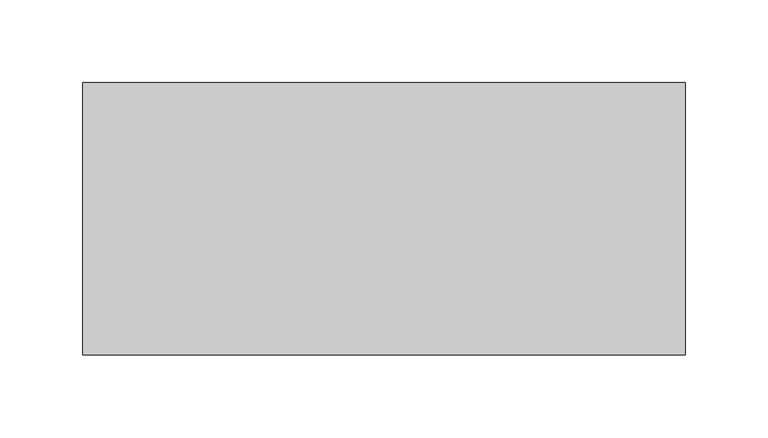
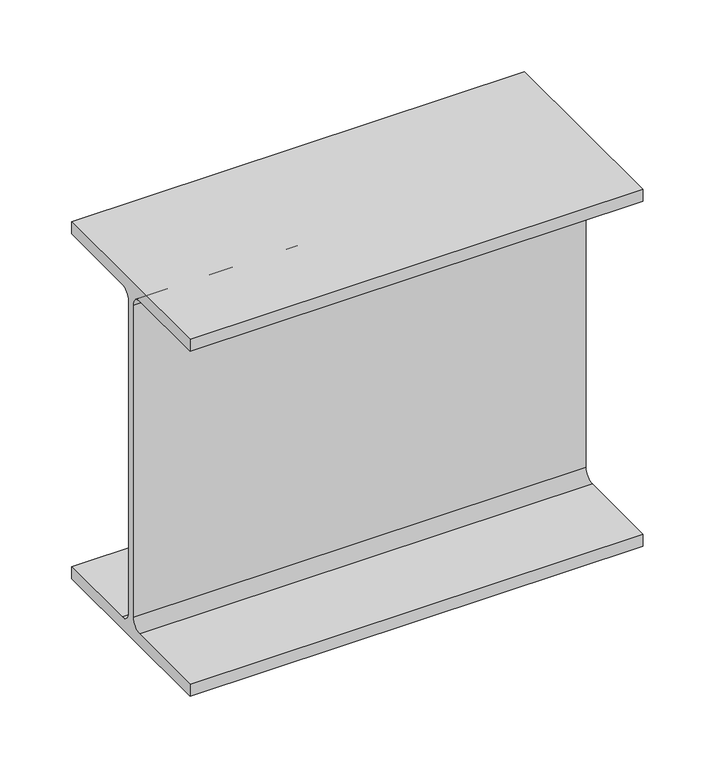
"""IFC4 building model written with IfcOpenShell, lengths in millimetres: beam geometry, Old_Steel Beam_H-KSD3502 : H_SB_ASB_H-300×150x6.5x9."""

import ifcopenshell
import ifcopenshell.guid

model = None  # the IFC model being written
_history = None  # IfcOwnerHistory: only IFC2X3 demands one
_inside = {}  # id of a spatial element -> (the spatial element, [elements in it])
_under = {}  # id of a project, library or spatial element -> (it, [spatial elements below it])
_declared = {}  # id of a project -> (the project, [libraries it declares])
_typed = {}  # id of a type object -> (the type object, [elements of that type])
_made_of = {}  # id of a material, layer set ... -> (it, [elements and type objects made of it])


def new_model(schema):
    """Start an empty IFC model of exactly this schema.

    Asked for "IFC4X3", IfcOpenShell would pick the latest addendum, in which some entities
    have other attributes; the version numbers below select the first issue.
    IFC2X3 requires an IfcOwnerHistory on every rooted entity: one is made here for all.
    """
    global model, _history
    if schema == "IFC4X3":
        model = ifcopenshell.file(schema_version=(4, 3, 0, 0))
    else:
        model = ifcopenshell.file(schema=schema)
    _inside.clear()
    _under.clear()
    _declared.clear()
    _typed.clear()
    _made_of.clear()
    _history = None
    if model.schema == "IFC2X3":
        org = make("IfcOrganization", Name="unknown")
        user = make(
            "IfcPersonAndOrganization",
            ThePerson=make("IfcPerson", FamilyName="unknown"),
            TheOrganization=org,
        )
        app = make(
            "IfcApplication",
            ApplicationDeveloper=org,
            Version="unknown",
            ApplicationFullName="unknown",
            ApplicationIdentifier="unknown",
        )
        _history = make(
            "IfcOwnerHistory",
            OwningUser=user,
            OwningApplication=app,
            ChangeAction="ADDED",
            CreationDate=0,
        )
    return model


def make(cls, **values):
    """One entity of the class cls with the attributes given. An attribute that is None is left unset."""
    return model.create_entity(
        cls, **{name: value for name, value in values.items() if value is not None}
    )


def rooted(cls, **values):
    """An entity with a GlobalId (a new one), such as an element, a storey or a relation."""
    return make(cls, GlobalId=ifcopenshell.guid.new(), OwnerHistory=_history, **values)


def si_unit(unit_type, name, prefix=None):
    """IfcSIUnit, for example si_unit("LENGTHUNIT", "METRE", prefix="MILLI")."""
    return make("IfcSIUnit", UnitType=unit_type, Prefix=prefix, Name=name)


def assignment(units):
    """IfcUnitAssignment: the units of a project."""
    return None if units is None else make("IfcUnitAssignment", Units=units)


def point(xyz):
    """IfcCartesianPoint."""
    return None if xyz is None else make("IfcCartesianPoint", Coordinates=xyz)


def direction(xyz):
    """IfcDirection."""
    return None if xyz is None else make("IfcDirection", DirectionRatios=xyz)


def frame(location, z_axis=None, x_axis=None):
    """IfcAxis2Placement3D, a coordinate frame: its origin and axes. An axis left out is left unset."""
    return make(
        "IfcAxis2Placement3D",
        Location=point(location),
        Axis=direction(z_axis),
        RefDirection=direction(x_axis),
    )


def frame_2d(location, x_axis=None):
    """IfcAxis2Placement2D, a coordinate frame in the plane: its origin and x axis."""
    return make(
        "IfcAxis2Placement2D", Location=point(location), RefDirection=direction(x_axis)
    )


def origin():
    """The frame at (0, 0, 0) with its axes left unset."""
    return frame((0.0, 0.0, 0.0))


def place(relative_to, where):
    """IfcLocalPlacement: puts the frame where relative to a parent placement (None: the world)."""
    return make(
        "IfcLocalPlacement", PlacementRelTo=relative_to, RelativePlacement=where
    )


def context(
    kind, dimensions, precision=None, world=None, true_north=None, identifier=None
):
    """IfcGeometricRepresentationContext, for example the 3D "Model" context."""
    return make(
        "IfcGeometricRepresentationContext",
        ContextIdentifier=identifier,
        ContextType=kind,
        CoordinateSpaceDimension=dimensions,
        Precision=precision,
        WorldCoordinateSystem=world,
        TrueNorth=true_north,
    )


def project(units=None, contexts=None):
    """IfcProject with its units and contexts."""
    return rooted(
        "IfcProject",
        Name="project",
        RepresentationContexts=contexts,
        UnitsInContext=assignment(units),
    )


def spatial(cls, under=None, at=None, **own):
    """A site, building, storey or space (cls), placed at a placement, below another one or the project."""
    s = rooted(cls, ObjectPlacement=at, **own)
    if under is not None:
        _under.setdefault(under.id(), (under, []))[1].append(s)
    return s


def polyline(points):
    """IfcPolyline through the points."""
    return make("IfcPolyline", Points=[point(p) for p in points])


def circle_curve(where, radius):
    """IfcCircle in the frame where."""
    return make("IfcCircle", Position=where, Radius=radius)


def trimmed(basis, trim1, trim2, sense, master):
    """IfcTrimmedCurve: the piece of a basis curve between two trims."""
    return make(
        "IfcTrimmedCurve",
        BasisCurve=basis,
        Trim1=trim1,
        Trim2=trim2,
        SenseAgreement=sense,
        MasterRepresentation=master,
    )


def segment(curve, same_sense, transition):
    """IfcCompositeCurveSegment."""
    return make(
        "IfcCompositeCurveSegment",
        Transition=transition,
        SameSense=same_sense,
        ParentCurve=curve,
    )


def composite_curve(segments, self_intersect=None):
    """IfcCompositeCurve: segments joined end to end."""
    return make("IfcCompositeCurve", Segments=segments, SelfIntersect=self_intersect)


def outline(outer, holes=None, kind="AREA"):
    """IfcArbitraryClosedProfileDef: a profile drawn as a closed curve; with holes, ...WithVoids."""
    if holes is None:
        return make("IfcArbitraryClosedProfileDef", ProfileType=kind, OuterCurve=outer)
    return make(
        "IfcArbitraryProfileDefWithVoids",
        ProfileType=kind,
        OuterCurve=outer,
        InnerCurves=holes,
    )


def extrude(swept, where, along, depth):
    """IfcExtrudedAreaSolid: the profile swept, set in the frame where, extruded along a direction by depth."""
    return make(
        "IfcExtrudedAreaSolid",
        SweptArea=swept,
        Position=where,
        ExtrudedDirection=direction(along),
        Depth=depth,
    )


def shape(context_of_items, identifier, shape_type, items):
    """IfcShapeRepresentation: the items that make up one representation, for example the "Body"."""
    return make(
        "IfcShapeRepresentation",
        ContextOfItems=context_of_items,
        RepresentationIdentifier=identifier,
        RepresentationType=shape_type,
        Items=items,
    )


def source(mapping_origin, context_of_items, identifier, shape_type, items):
    """IfcRepresentationMap: a shape defined once, which mapped items show again and again."""
    return make(
        "IfcRepresentationMap",
        MappingOrigin=mapping_origin,
        MappedRepresentation=shape(context_of_items, identifier, shape_type, items),
    )


def transform(
    local_origin,
    x_axis=None,
    y_axis=None,
    z_axis=None,
    scale=None,
    scale2=None,
    scale3=None,
    uniform=True,
):
    """IfcCartesianTransformationOperator3D, or its non-uniform kind. x_axis, y_axis, z_axis: its Axis1, 2, 3."""
    if uniform:
        return make(
            "IfcCartesianTransformationOperator3D",
            Axis1=direction(x_axis),
            Axis2=direction(y_axis),
            LocalOrigin=point(local_origin),
            Scale=scale,
            Axis3=direction(z_axis),
        )
    return make(
        "IfcCartesianTransformationOperator3DnonUniform",
        Axis1=direction(x_axis),
        Axis2=direction(y_axis),
        LocalOrigin=point(local_origin),
        Scale=scale,
        Axis3=direction(z_axis),
        Scale2=scale2,
        Scale3=scale3,
    )


def mapped(mapping_source, mapping_target):
    """IfcMappedItem: shows the shape of a source again, moved by a transform."""
    return make(
        "IfcMappedItem", MappingSource=mapping_source, MappingTarget=mapping_target
    )


def made_of(thing, what):
    """Note that an element or type object is made of a material, layer set ...; save() writes the relation."""
    if what is not None:
        _made_of.setdefault(what.id(), (what, []))[1].append(thing)
    return thing


def element(
    cls,
    number,
    at=None,
    inside=None,
    cuts=None,
    type_object=None,
    material=None,
    context=None,
    identifier="Body",
    shape_type=None,
    held_by="IfcProductDefinitionShape",
    body=None,
    shapes=None,
    **own,
):
    """One element of the class cls, such as IfcWall. Its Tag is "e" and its number.

    at: its placement. inside: the storey or other place that contains it. cuts: it is an
    opening in that element (IfcRelVoidsElement). A single representation is given by context,
    identifier, shape_type and body (its items); several are given by shapes. held_by: the class
    of the entity that holds the representations. save() writes the other relations.
    """
    e = rooted(cls, Tag="e%d" % number, ObjectPlacement=at, **own)
    if body is not None:
        shapes = [shape(context, identifier, shape_type, body)]
    if shapes is not None:
        e.Representation = make(held_by, Representations=shapes)
    if inside is not None:
        _inside.setdefault(inside.id(), (inside, []))[1].append(e)
    if cuts is not None:
        rooted(
            "IfcRelVoidsElement", RelatingBuildingElement=cuts, RelatedOpeningElement=e
        )
    if type_object is not None:
        _typed.setdefault(type_object.id(), (type_object, []))[1].append(e)
    return made_of(e, material)


def aggregate(whole, parts):
    """IfcRelAggregates: a whole, such as a stair, and the parts it consists of."""
    return rooted("IfcRelAggregates", RelatingObject=whole, RelatedObjects=parts)


def save(model, path):
    """Write the relations noted so far, then the file.

    IfcRelAggregates (storeys below a building ...), IfcRelContainedInSpatialStructure (elements
    in a storey), IfcRelDefinesByType, IfcRelAssociatesMaterial and IfcRelDeclares: one each for
    every whole, place, type object, material and project.
    """
    for whole, parts in _under.values():
        aggregate(whole, parts)
    for where, things in _inside.values():
        rooted(
            "IfcRelContainedInSpatialStructure",
            RelatedElements=things,
            RelatingStructure=where,
        )
    for kind, things in _typed.values():
        rooted("IfcRelDefinesByType", RelatedObjects=things, RelatingType=kind)
    for what, things in _made_of.values():
        rooted("IfcRelAssociatesMaterial", RelatedObjects=things, RelatingMaterial=what)
    for by, libraries in _declared.values():
        rooted("IfcRelDeclares", RelatingContext=by, RelatedDefinitions=libraries)
    model.write(path)


def beam_05e9ef29(model_context):
    return source(origin(), model_context, "Body", "SweptSolid", [
        extrude(outline(composite_curve([segment(polyline([(82.5, -141.5), (82.5, -151.7), (-82.5, -151.7), (-82.5, -141.5), (-11.9, -141.5)]), True, "CONTINUOUS"), segment(trimmed(circle_curve(frame_2d((-11.9, -132.6)), 8.9), [point((-11.9, -141.5))], [point((-3.0, -132.6))], True, "CARTESIAN"), True, "CONTINUOUS"), segment(polyline([(-3.0, -132.6), (-3.0, 132.6)]), True, "CONTINUOUS"), segment(trimmed(circle_curve(frame_2d((-11.9, 132.6)), 8.9), [point((-3.0, 132.6))], [point((-11.9, 141.5))], True, "CARTESIAN"), True, "CONTINUOUS"), segment(polyline([(-11.9, 141.5), (-82.5, 141.5), (-82.5, 151.7), (82.5, 151.7), (82.5, 141.5), (11.9, 141.5)]), True, "CONTINUOUS"), segment(trimmed(circle_curve(frame_2d((11.9, 132.6)), 8.9), [point((11.9, 141.5))], [point((3.0, 132.6))], True, "CARTESIAN"), True, "CONTINUOUS"), segment(polyline([(3.0, 132.6), (3.0, -132.6)]), True, "CONTINUOUS"), segment(trimmed(circle_curve(frame_2d((11.9, -132.6)), 8.9), [point((3.0, -132.6))], [point((11.9, -141.5))], True, "CARTESIAN"), True, "CONTINUOUS"), segment(polyline([(11.9, -141.5), (82.5, -141.5)]), True, "CONTINUOUS")], self_intersect=False)), frame((-107.3, 0.0, 0.0), z_axis=(1.0, 0.0, 0.0), x_axis=(0.0, 1.0, 0.0)), (0.0, 0.0, 1.0), 364.5999994),
    ])


if __name__ == "__main__":
    model = new_model("IFC4")
    model_context = context("Model", 3, world=origin())
    ifc_project = project(units=[si_unit("LENGTHUNIT", "METRE", prefix="MILLI")], contexts=[model_context])
    site = spatial("IfcSite", under=ifc_project)
    building = spatial("IfcBuilding", under=site)
    placement = place(None, origin())
    beam_shape = beam_05e9ef29(model_context)
    element("IfcBeam", 1, ObjectType="Old_Steel Beam_H-KSD3502 : H_SB_ASB_H-300×150x6.5x9", at=placement, inside=building, context=model_context, shape_type="MappedRepresentation", body=[
        mapped(beam_shape, transform((0.0, 0.0, 0.0), x_axis=(1.0, 0.0, 0.0), y_axis=(0.0, 1.0, 0.0), z_axis=(0.0, 0.0, 1.0))),
    ])
    save(model, "model.ifc")

# Revit data of these elements
# Project information
#   Building Name = "STEAM TURBINE BUILDING"
#   Project Status = "Project Status"
#   Client Name = "현대엔지니어링"
#   Project Address = "서울시 종로구 율곡로 75(계동)"
#   Project Name = "Therma Visayas Energy Project"
#   Project Number = "-"
# Type "Old_Steel Beam_H-KSD3502 : H_SB_ASB_H-300×150x6.5x9"
#   Width = 15.0 cm
#   Web Thickness = 0.65 cm
#   Web Fillet = 1.3 cm
#   Warping Constant = 107174.0 cm⁶
#   Torsional Moment of Inertia = 9.9539 cm⁴
#   Torsional Modulus = 1.0 cm³
#   Section Area = 46.78 cm²
#   Plastic Modulus weak axis = 105.0 cm³
#   Plastic Modulus strong axis = 542.0 cm³
#   Perimeter = 1.17 m²/m
#   Nominal Weight = 36.70 kgf/m
#   Moment of Inertia weak axis = 508.00 cm⁴
#   Moment of Inertia strong axis = 7210.00 cm⁴
#   Height = 30.0 cm
#   Flange Thickness = 0.9 cm
#   Elastic Modulus weak axis = 67.7 cm³
#   Elastic Modulus strong axis = 481.0 cm³
#   Centroid Vertical = 15.0 cm
#   Centroid Horizontal = 7.5 cm
#   Length [instance default] = 1.5240 m
#   Structural Material [instance default] = Steel, 45-345
#   Assembly Code = ""
# Element 1 (IfcBeam, "Old_Steel Beam_H-KSD3502 : H_SB_ASB_H-300×150x6.5x9")
#   Structural Material = none
# Materials
#   "Steel, 45-345": class "Metal", colour RGB 189 187 185, transparency 0, Description = "Steel 345 MPa", Cost = 0
